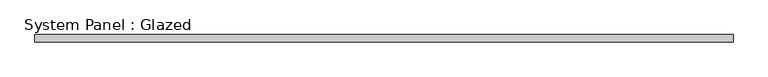
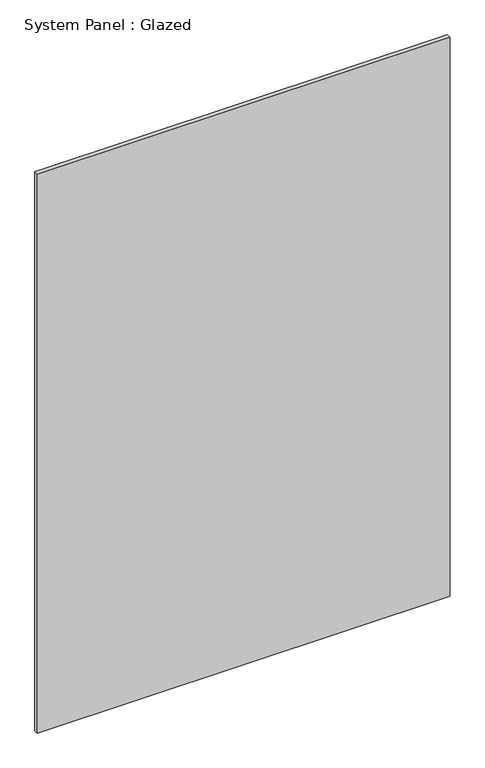
"""IFC4 building model written with IfcOpenShell, lengths in millimetres: plate geometry, System Panel : Glazed."""

from ifc_helpers import new_model, si_unit, origin, origin_with_axes, place, context, project, spatial, polyline, outline, extrude, source, transform, mapped, element, save


def system_panel_glazed_15c79043(model_context):
    return source(origin(), model_context, "Body", "SweptSolid", [
        extrude(outline(polyline([(1177.8211268, 24.5), (-1177.8211268, 24.5), (-1177.8211268, 49.5), (1177.8211268, 49.5), (1177.8211268, 24.5)])), origin_with_axes(), (0.0, 0.0, 1.0), 3370.0),
    ])


if __name__ == "__main__":
    model = new_model("IFC4")
    model_context = context("Model", 3, world=origin())
    ifc_project = project(units=[si_unit("LENGTHUNIT", "METRE", prefix="MILLI")], contexts=[model_context])
    site = spatial("IfcSite", under=ifc_project)
    building = spatial("IfcBuilding", under=site)
    placement = place(None, origin())
    system_panel_glazed_shape = system_panel_glazed_15c79043(model_context)
    element("IfcPlate", 1, ObjectType="System Panel : Glazed", at=placement, inside=building, context=model_context, shape_type="MappedRepresentation", body=[
        mapped(system_panel_glazed_shape, transform((0.0, 0.0, 0.0), x_axis=(1.0, 0.0, 0.0), y_axis=(0.0, 1.0, 0.0), z_axis=(0.0, 0.0, 1.0))),
    ])
    save(model, "model.ifc")

# Revit data of these elements
# Type "System Panel : Glazed"
#   Construction Type Id = "GSP4R"
#   Analytic Construction = "1/8 in Pilkington single glazing"
#   Visual Light Transmittance = 0.9
#   Solar Heat Gain Coefficient = 0.86
#   Heat Transfer Coefficient (U) = 6.7069 W/(m²·K)
#   Define Thermal Properties by = 1
# Element 1 (IfcPlate, "System Panel : Glazed")
#   Materials on its faces: "Glass"
# Materials
#   "Glass": class "Glass", colour RGB 245 245 243, transparency 1, Description = "Soda Lime Glass", Cost = 0
